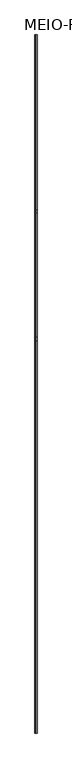
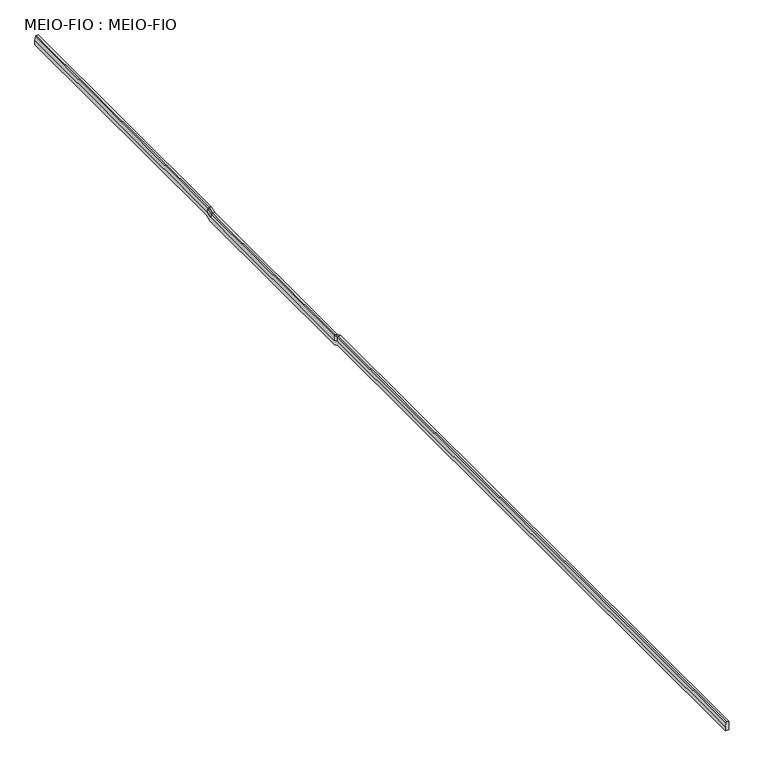
"""IFC4 building model written with IfcOpenShell, lengths in millimetres: proxy geometry, MEIO-FIO : MEIO-FIO."""

from ifc_helpers import new_model, si_unit, frame, origin, place, context, project, spatial, circle_curve, ellipse_curve, source, transform, mapped, element, save
from ifc_brep_helpers import plane_surface, cylinder_surface, advanced_brep


def meio_fio_meio_fio_c5939b1e(model_context):
    return source(origin(), model_context, "Body", "AdvancedBrep", [
        advanced_brep(
        [(-19460.281307, 17327.5225294, 100.0), (-19460.281307, 17327.5225294, -200.0), (-19580.281307, 17327.5225294, -200.0), (-19580.281307, 17327.5225294, -50.0), (-19560.334366, 17327.5225294, 74.7371665), (-19530.7107394, 17327.5225294, 100.0), (-19460.281307, 7304.4300153, 100.0), (-19460.281307, 7104.4300153, 20.0), (-19460.281307, 4.4300153, 20.0), (-19460.281307, -195.5699847, 100.0), (-19460.281307, -22700.938406, 100.0), (-19460.281307, -22700.938406, -200.0), (-19460.281307, -253.3447058, -200.0), (-19460.281307, -53.3447058, -280.0), (-19460.281307, 7162.2047364, -280.0), (-19460.281307, 7362.2047364, -200.0), (-19580.281307, 7362.2047364, -200.0), (-19580.281307, 7162.2047364, -280.0), (-19580.281307, -53.3447058, -280.0), (-19580.281307, -253.3447058, -200.0), (-19580.281307, -22700.938406, -200.0), (-19580.281307, -22700.938406, -50.0), (-19580.281307, -224.4573452, -50.0), (-19580.281307, -24.4573452, -130.0), (-19580.281307, 7133.3173758, -130.0), (-19580.281307, 7333.3173758, -50.0), (-19560.334366, 7309.2951925, 74.7371665), (-19530.7107394, 7304.4300153, 100.0), (-19560.334366, 7109.2951925, -5.2628335), (-19530.7107394, 7104.4300153, 20.0), (-19560.334366, -0.4351619, -5.2628335), (-19530.7107394, 4.4300153, 20.0), (-19560.334366, -200.4351619, 74.7371665), (-19530.7107394, -195.5699847, 100.0), (-19530.7107394, -22700.938406, 100.0), (-19560.334366, -22700.938406, 74.7371665)],
        [
            (0, 1),
            (1, 2),
            (2, 3),
            (3, 4),
            (4, 5, circle_curve(frame((-19530.7107394, 17327.5225294, 70.0), z_axis=(0.0, 1.0, 0.0), x_axis=(-1.0, 0.0, 0.0)), 30.0)),
            (5, 0),
            (0, 6),
            (6, 7),
            (7, 8),
            (8, 9),
            (9, 10),
            (10, 11),
            (11, 12),
            (12, 13),
            (13, 14),
            (14, 15),
            (15, 1),
            (15, 16),
            (16, 2),
            (16, 17),
            (17, 18),
            (18, 19),
            (19, 20),
            (20, 21),
            (21, 22),
            (22, 23),
            (23, 24),
            (24, 25),
            (25, 3),
            (25, 26),
            (26, 4),
            (26, 27, ellipse_curve(frame((-19530.7107394, 7310.2074874, 70.0), z_axis=(0.0, 0.9819563867314226, 0.18910752115494767), x_axis=(0.0, 0.18910752115494667, -0.9819563867314226)), 30.551255, 30.0)),
            (27, 5),
            (27, 6),
            (14, 17),
            (24, 28),
            (28, 26),
            (28, 29, ellipse_curve(frame((-19530.7107394, 7110.2074874, -10.0), z_axis=(0.0, 0.9819563867314226, 0.18910752115494764), x_axis=(0.0, -0.18910752115494842, 0.9819563867314223)), 30.551255, 30.0)),
            (29, 27),
            (29, 7),
            (13, 18),
            (23, 30),
            (30, 28),
            (30, 31, ellipse_curve(frame((-19530.7107394, -1.3474568, -10.0), z_axis=(0.0, 0.9819563867314217, -0.1891075211549513), x_axis=(0.0, 0.18910752115495252, 0.9819563867314217)), 30.551255, 30.0)),
            (31, 29),
            (31, 8),
            (12, 19),
            (22, 32),
            (32, 30),
            (32, 33, ellipse_curve(frame((-19530.7107394, -201.3474568, 70.0), z_axis=(0.0, 0.9819563867314217, -0.18910752115495139), x_axis=(0.0, -0.18910752115495078, -0.9819563867314218)), 30.551255, 30.0)),
            (33, 31),
            (33, 9),
            (10, 34),
            (34, 35, circle_curve(frame((-19530.7107394, -22700.938406, 70.0), z_axis=(0.0, -1.0, 0.0), x_axis=(-1.0, 0.0, 0.0)), 30.0)),
            (35, 21),
            (20, 11),
            (35, 32),
            (34, 33),
        ],
        [
            plane_surface(frame((-19460.281307, 17327.5225294, 100.0), z_axis=(0.0, 1.0, 0.0), x_axis=(0.0, 0.0, 1.0))),
            plane_surface(frame((-19460.281307, 17327.5225294, 100.0), z_axis=(1.0, 0.0, 0.0), x_axis=(0.0, -1.0, 0.0))),
            plane_surface(frame((-19460.281307, 17327.5225294, -200.0), z_axis=(0.0, 0.0, -1.0), x_axis=(0.0, -1.0, 0.0))),
            plane_surface(frame((-19580.281307, 17327.5225294, -200.0), z_axis=(-1.0, 0.0, 0.0), x_axis=(0.0, -1.0, 0.0))),
            plane_surface(frame((-19580.281307, 17327.5225294, -50.0), z_axis=(-0.9874542202157147, 0.0, 0.15790555081495689), x_axis=(0.0, -1.0, 0.0))),
            cylinder_surface(frame((-19530.7107394, 17327.5225294, 70.0), z_axis=(0.0, 1.0, 0.0), x_axis=(-1.0, 0.0, 0.0)), 30.0),
            plane_surface(frame((-19530.7107394, 17327.5225294, 100.0), z_axis=(0.0, 0.0, 1.0), x_axis=(0.0, -1.0, 0.0))),
            plane_surface(frame((-19460.281307, 7362.2047364, -200.0), z_axis=(0.0, 0.3713906763540969, -0.9284766908852621), x_axis=(0.0, -0.9284766908852621, -0.3713906763540969))),
            plane_surface(frame((-19580.281307, 7333.3173758, -50.0), z_axis=(-0.9874542202157147, -0.05864464931723302, 0.1466116232930858), x_axis=(0.0, -0.9284766908852622, -0.3713906763540966))),
            cylinder_surface(frame((-19530.7107394, 7315.5717356, 72.1456993), z_axis=(0.0, 0.9284766908852621, 0.3713906763540969), x_axis=(-1.0, 0.0, 0.0)), 30.0),
            plane_surface(frame((-19530.7107394, 7304.4300153, 100.0), z_axis=(0.0, -0.37139067635409667, 0.9284766908852622), x_axis=(0.0, -0.9284766908852622, -0.37139067635409667))),
            plane_surface(frame((-19460.281307, 7162.2047364, -280.0), z_axis=(0.0, 0.0, -1.0), x_axis=(0.0, -1.0, 0.0))),
            plane_surface(frame((-19580.281307, 7133.3173758, -130.0), z_axis=(-0.9874542202157146, 0.0, 0.15790555081495686), x_axis=(0.0, -1.0, 0.0))),
            cylinder_surface(frame((-19530.7107394, 7104.4300153, -10.0), z_axis=(0.0, 1.0, 0.0), x_axis=(-1.0, 0.0, 0.0)), 30.0),
            plane_surface(frame((-19530.7107394, 7104.4300153, 20.0), z_axis=(0.0, 0.0, 1.0), x_axis=(0.0, -1.0, 0.0))),
            plane_surface(frame((-19460.281307, -53.3447058, -280.0), z_axis=(0.0, -0.37139067635410367, -0.9284766908852594), x_axis=(0.0, -0.9284766908852594, 0.37139067635410367))),
            plane_surface(frame((-19580.281307, -24.4573452, -130.0), z_axis=(-0.9874542202157147, 0.05864464931723411, 0.14661162329308536), x_axis=(0.0, -0.9284766908852594, 0.37139067635410355))),
            cylinder_surface(frame((-19530.7107394, -6.711705, -7.8543007), z_axis=(0.0, 0.9284766908852593, -0.3713906763541038), x_axis=(-1.0, 0.0, 0.0)), 30.0),
            plane_surface(frame((-19530.7107394, 4.4300153, 20.0), z_axis=(0.0, 0.3713906763541038, 0.9284766908852593), x_axis=(0.0, -0.9284766908852593, 0.3713906763541038))),
            plane_surface(frame((-19460.281307, -22700.938406, 100.0), z_axis=(0.0, -1.0, 0.0), x_axis=(0.0, 0.0, 1.0))),
            plane_surface(frame((-19460.281307, -253.3447058, -200.0), z_axis=(0.0, 0.0, -1.0), x_axis=(0.0, -1.0, 0.0))),
            plane_surface(frame((-19580.281307, -224.4573452, -50.0), z_axis=(-0.9874542202157146, 0.0, 0.15790555081495683), x_axis=(0.0, -1.0, 0.0))),
            cylinder_surface(frame((-19530.7107394, -195.5699847, 70.0), z_axis=(0.0, 1.0, 0.0), x_axis=(-1.0, 0.0, 0.0)), 30.0),
            plane_surface(frame((-19530.7107394, -195.5699847, 100.0), z_axis=(0.0, 0.0, 1.0), x_axis=(0.0, -1.0, 0.0))),
        ],
        [
            (0, [[1, 2, 3, 4, 5, 6]]),
            (1, [[-1, 7, 8, 9, 10, 11, 12, 13, 14, 15, 16, 17]]),
            (2, [[-2, -17, 18, 19]]),
            (3, [[-3, -19, 20, 21, 22, 23, 24, 25, 26, 27, 28, 29]]),
            (4, [[-4, -29, 30, 31]]),
            (5, [[-5, -31, 32, 33]]),
            (6, [[-6, -33, 34, -7]]),
            (7, [[-18, -16, 35, -20]]),
            (8, [[-30, -28, 36, 37]]),
            (9, [[-32, -37, 38, 39]]),
            (10, [[-34, -39, 40, -8]]),
            (11, [[-35, -15, 41, -21]]),
            (12, [[-36, -27, 42, 43]]),
            (13, [[-38, -43, 44, 45]]),
            (14, [[-40, -45, 46, -9]]),
            (15, [[-41, -14, 47, -22]]),
            (16, [[-42, -26, 48, 49]]),
            (17, [[-44, -49, 50, 51]]),
            (18, [[-46, -51, 52, -10]]),
            (19, [[53, 54, 55, -24, 56, -12]]),
            (20, [[-47, -13, -56, -23]]),
            (21, [[-48, -25, -55, 57]]),
            (22, [[-50, -57, -54, 58]]),
            (23, [[-52, -58, -53, -11]]),
        ],
    ),
    ])


if __name__ == "__main__":
    model = new_model("IFC4")
    model_context = context("Model", 3, world=origin())
    ifc_project = project(units=[si_unit("LENGTHUNIT", "METRE", prefix="MILLI")], contexts=[model_context])
    site = spatial("IfcSite", under=ifc_project)
    building = spatial("IfcBuilding", under=site)
    placement = place(None, origin())
    meio_fio_meio_fio_shape = meio_fio_meio_fio_c5939b1e(model_context)
    element("IfcBuildingElementProxy", 1, Name="MEIO-FIO : MEIO-FIO", ObjectType="MEIO-FIO : MEIO-FIO", at=placement, inside=building, context=model_context, shape_type="MappedRepresentation", body=[
        mapped(meio_fio_meio_fio_shape, transform((0.0, 0.0, 0.0), x_axis=(1.0, 0.0, 0.0), y_axis=(0.0, 1.0, 0.0), z_axis=(0.0, 0.0, 1.0))),
    ])
    save(model, "model.ifc")

# Revit data of these elements
# Element 1 (IfcBuildingElementProxy, "MEIO-FIO : MEIO-FIO")
#   Materials on its faces: ".PAVIMENTAÇÃO CALÇADA"
# Materials
#   ".PAVIMENTAÇÃO CALÇADA": class ".CC_PAVIMENTAÇÃO", colour RGB 176 176 176, transparency 0, Description = "Pavimentação calçada cinza claro", Cost = 0
